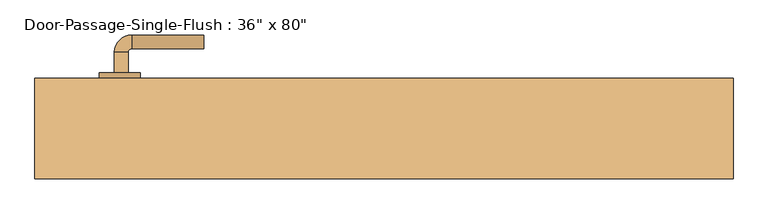
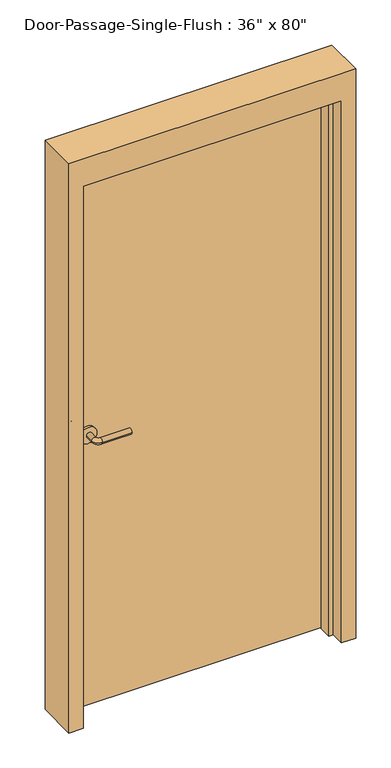
"""IFC4 building model written with IfcOpenShell, lengths in millimetres: door geometry."""

from ifc_helpers import new_model, si_unit, point, frame, frame_2d, origin, origin_with_axes, place, context, project, spatial, polyline, circle_curve, ellipse_curve, trimmed, segment, composite_curve, outline, extrude, faceted_brep, source, transform, mapped, element, save
from ifc_brep_helpers import plane_surface, cylinder_surface, revolved_surface, advanced_brep


def door_64a1d9e0(model_context):
    return source(origin(), model_context, "Body", "SolidModel", [
        advanced_brep(
        [(-392.190625, 17.4, 1016.0), (-372.190625, 17.4, 1016.0), (-372.190625, -12.6, 1016.0), (-392.190625, -12.6, 1016.0), (-367.190625, -17.6, 1016.0), (-367.190625, -37.6, 1016.0), (-262.190625, -37.6, 1016.0), (-262.190625, -17.6, 1016.0)],
        [
            (0, 1, circle_curve(frame((-382.190625, 17.4, 1016.0), z_axis=(0.0, 1.0, 0.0), x_axis=(1.0, 0.0, 0.0)), 10.0)),
            (1, 0, circle_curve(frame((-382.190625, 17.4, 1016.0), z_axis=(0.0, 1.0, 0.0), x_axis=(1.0, 0.0, 0.0)), 10.0)),
            (1, 2),
            (2, 3, circle_curve(frame((-382.190625, -12.6, 1016.0), z_axis=(0.0, 1.0, 0.0), x_axis=(1.0, 0.0, 0.0)), 10.0)),
            (3, 0),
            (3, 2, circle_curve(frame((-382.190625, -12.6, 1016.0), z_axis=(0.0, 1.0, 0.0), x_axis=(1.0, 0.0, 0.0)), 10.0)),
            (4, 5, circle_curve(frame((-367.190625, -27.6, 1016.0), z_axis=(-1.0, 0.0, 0.0), x_axis=(0.0, 1.0, 0.0)), 10.0)),
            (5, 3, circle_curve(frame((-367.190625, -12.6, 1016.0), z_axis=(0.0, 0.0, -1.0), x_axis=(-1.0, 0.0, 0.0)), 25.0)),
            (2, 4, circle_curve(frame((-367.190625, -12.6, 1016.0), z_axis=(0.0, 0.0, 1.0), x_axis=(-1.0, 0.0, 0.0)), 5.0)),
            (5, 4, circle_curve(frame((-367.190625, -27.6, 1016.0), z_axis=(-1.0, 0.0, 0.0), x_axis=(0.0, 1.0, 0.0)), 10.0)),
            (6, 7, circle_curve(frame((-262.190625, -27.6, 1016.0), z_axis=(1.0, 0.0, 0.0), x_axis=(0.0, 1.0, 0.0)), 10.0)),
            (7, 6, circle_curve(frame((-262.190625, -27.6, 1016.0), z_axis=(1.0, 0.0, 0.0), x_axis=(0.0, 1.0, 0.0)), 10.0)),
            (4, 7),
            (6, 5),
        ],
        [
            plane_surface(frame((-382.190625, 17.4, 1016.0), z_axis=(0.0, 1.0, 0.0), x_axis=(0.0, 0.0, 1.0))),
            cylinder_surface(frame((-382.190625, 17.4, 1016.0), z_axis=(0.0, 1.0, 0.0), x_axis=(1.0, 0.0, 0.0)), 10.0),
            revolved_surface(trimmed(ellipse_curve(frame((-382.190625, -12.6, 1016.0), z_axis=(0.0, -1.0, 0.0), x_axis=(1.0, 0.0, 0.0)), 10.0, 10.0), [point((-392.190625, -12.6, 1016.0))], [point((-372.190625, -12.6, 1016.0))], True, "CARTESIAN"), (-367.190625, -12.6, 1016.0), (0.0, 0.0, -1.0)),
            revolved_surface(trimmed(ellipse_curve(frame((-382.190625, -12.6, 1016.0), z_axis=(0.0, -1.0, 0.0), x_axis=(1.0, 0.0, 0.0)), 10.0, 10.0), [point((-372.190625, -12.6, 1016.0))], [point((-392.190625, -12.6, 1016.0))], True, "CARTESIAN"), (-367.190625, -12.6, 1016.0), (0.0, 0.0, -1.0)),
            plane_surface(frame((-262.190625, -27.6, 1016.0), z_axis=(1.0, 0.0, 0.0), x_axis=(0.0, 0.0, 1.0))),
            cylinder_surface(frame((-367.190625, -27.6, 1016.0), z_axis=(-1.0, 0.0, 0.0), x_axis=(0.0, 1.0, 0.0)), 10.0),
        ],
        [
            (0, [[1, 2]]),
            (1, [[3, 4, 5, -2]]),
            (1, [[-5, 6, -3, -1]]),
            (2, [[7, 8, -4, 9]]),
            (3, [[10, -9, -6, -8]]),
            (4, [[11, 12]]),
            (5, [[13, -11, 14, -7]]),
            (5, [[-14, -12, -13, -10]]),
        ],
    ),
        extrude(outline(composite_curve([segment(trimmed(circle_curve(frame_2d((1016.0, -384.690625)), 30.0), [point((1016.0, -414.690625))], [point((1016.0, -354.690625))], False, "CARTESIAN"), True, "CONTINUOUS"), segment(trimmed(circle_curve(frame_2d((1016.0, -384.690625)), 30.0), [point((1016.0, -354.690625))], [point((1016.0, -414.690625))], False, "CARTESIAN"), True, "CONTINUOUS")], self_intersect=False)), frame((0.0, 17.4, 0.0), z_axis=(0.0, 1.0, 0.0), x_axis=(0.0, 0.0, 1.0)), (0.0, 0.0, 1.0), 8.0),
        advanced_brep(
        [(-392.190625, 77.85, 1016.0), (-372.190625, 77.85, 1016.0), (-392.190625, 107.85, 1016.0), (-372.190625, 107.85, 1016.0), (-367.190625, 112.85, 1016.0), (-367.190625, 132.85, 1016.0), (-262.190625, 132.85, 1016.0), (-262.190625, 112.85, 1016.0)],
        [
            (0, 1, circle_curve(frame((-382.190625, 77.85, 1016.0), z_axis=(0.0, -1.0, 0.0), x_axis=(1.0, 0.0, 0.0)), 10.0)),
            (1, 0, circle_curve(frame((-382.190625, 77.85, 1016.0), z_axis=(0.0, -1.0, 0.0), x_axis=(1.0, 0.0, 0.0)), 10.0)),
            (0, 2),
            (2, 3, circle_curve(frame((-382.190625, 107.85, 1016.0), z_axis=(0.0, -1.0, 0.0), x_axis=(1.0, 0.0, 0.0)), 10.0)),
            (3, 1),
            (3, 2, circle_curve(frame((-382.190625, 107.85, 1016.0), z_axis=(0.0, -1.0, 0.0), x_axis=(1.0, 0.0, 0.0)), 10.0)),
            (4, 3, circle_curve(frame((-367.190625, 107.85, 1016.0), z_axis=(0.0, 0.0, 1.0), x_axis=(-1.0, 0.0, 0.0)), 5.0)),
            (2, 5, circle_curve(frame((-367.190625, 107.85, 1016.0), z_axis=(0.0, 0.0, -1.0), x_axis=(-1.0, 0.0, 0.0)), 25.0)),
            (5, 4, circle_curve(frame((-367.190625, 122.85, 1016.0), z_axis=(-1.0, 0.0, 0.0), x_axis=(0.0, -1.0, 0.0)), 10.0)),
            (4, 5, circle_curve(frame((-367.190625, 122.85, 1016.0), z_axis=(-1.0, 0.0, 0.0), x_axis=(0.0, -1.0, 0.0)), 10.0)),
            (6, 7, circle_curve(frame((-262.190625, 122.85, 1016.0), z_axis=(1.0, 0.0, 0.0), x_axis=(0.0, -1.0, 0.0)), 10.0)),
            (7, 6, circle_curve(frame((-262.190625, 122.85, 1016.0), z_axis=(1.0, 0.0, 0.0), x_axis=(0.0, -1.0, 0.0)), 10.0)),
            (5, 6),
            (7, 4),
        ],
        [
            plane_surface(frame((-382.190625, 77.85, 1016.0), z_axis=(0.0, -1.0, 0.0), x_axis=(0.0, 0.0, 1.0))),
            cylinder_surface(frame((-382.190625, 77.85, 1016.0), z_axis=(0.0, -1.0, 0.0), x_axis=(1.0, 0.0, 0.0)), 10.0),
            revolved_surface(trimmed(ellipse_curve(frame((-382.190625, 107.85, 1016.0), z_axis=(0.0, -1.0, 0.0), x_axis=(1.0, 0.0, 0.0)), 10.0, 10.0), [point((-392.190625, 107.85, 1016.0))], [point((-372.190625, 107.85, 1016.0))], True, "CARTESIAN"), (-367.190625, 107.85, 1016.0), (0.0, 0.0, -1.0)),
            revolved_surface(trimmed(ellipse_curve(frame((-382.190625, 107.85, 1016.0), z_axis=(0.0, -1.0, 0.0), x_axis=(1.0, 0.0, 0.0)), 10.0, 10.0), [point((-372.190625, 107.85, 1016.0))], [point((-392.190625, 107.85, 1016.0))], True, "CARTESIAN"), (-367.190625, 107.85, 1016.0), (0.0, 0.0, -1.0)),
            plane_surface(frame((-262.190625, 122.85, 1016.0), z_axis=(1.0, 0.0, 0.0), x_axis=(0.0, 0.0, 1.0))),
            cylinder_surface(frame((-367.190625, 122.85, 1016.0), z_axis=(-1.0, 0.0, 0.0), x_axis=(0.0, -1.0, 0.0)), 10.0),
        ],
        [
            (0, [[1, 2]]),
            (1, [[-1, 3, 4, 5]]),
            (1, [[-2, -5, 6, -3]]),
            (2, [[7, -4, 8, 9]]),
            (3, [[-8, -6, -7, 10]]),
            (4, [[11, 12]]),
            (5, [[-9, 13, -12, 14]]),
            (5, [[-10, -14, -11, -13]]),
        ],
    ),
        extrude(outline(composite_curve([segment(trimmed(circle_curve(frame_2d((1016.0, -384.690625)), 30.0), [point((1016.0, -414.690625))], [point((1016.0, -354.690625))], False, "CARTESIAN"), True, "CONTINUOUS"), segment(trimmed(circle_curve(frame_2d((1016.0, -384.690625)), 30.0), [point((1016.0, -354.690625))], [point((1016.0, -414.690625))], False, "CARTESIAN"), True, "CONTINUOUS")], self_intersect=False)), frame((0.0, 69.85, 0.0), z_axis=(0.0, 1.0, 0.0), x_axis=(0.0, 0.0, 1.0)), (0.0, 0.0, 1.0), 8.0),
        faceted_brep([(457.2, 20.6375, 0.0), (457.2, 69.85, 0.0), (508.0, 69.85, 0.0), (508.0, -76.2, 0.0), (457.2, -76.2, 0.0), (457.2, -26.9875, 0.0), (441.325, -26.9875, 0.0), (441.325, 20.6375, 0.0), (457.2, 20.6375, 2032.0), (457.2, 69.85, 2032.0), (-457.2, 69.85, 2032.0), (-457.2, 69.85, 0.0), (-508.0, 69.85, 0.0), (-508.0, 69.85, 2133.6), (508.0, 69.85, 2133.6), (508.0, -76.2, 2133.6), (-508.0, -76.2, 2133.6), (-508.0, -76.2, 0.0), (-457.2, -76.2, 0.0), (-457.2, -76.2, 2032.0), (457.2, -76.2, 2032.0), (457.2, -26.9875, 2032.0), (-457.2, -26.9875, 2032.0), (-457.2, -26.9875, 0.0), (-441.325, -26.9875, 0.0), (-441.325, -26.9875, 2016.125), (441.325, -26.9875, 2016.125), (441.325, 20.6375, 2016.125), (-441.325, 20.6375, 2016.125), (-441.325, 20.6375, 0.0), (-457.2, 20.6375, 0.0), (-457.2, 20.6375, 2032.0)], [[[0, 1, 2, 3, 4, 5, 6, 7]], [[1, 0, 8, 9]], [[2, 1, 9, 10, 11, 12, 13, 14]], [[3, 2, 14, 15]], [[4, 3, 15, 16, 17, 18, 19, 20]], [[5, 4, 20, 21]], [[6, 5, 21, 22, 23, 24, 25, 26]], [[7, 6, 26, 27]], [[0, 7, 27, 28, 29, 30, 31, 8]], [[9, 8, 31, 10]], [[20, 19, 22, 21]], [[26, 25, 28, 27]], [[12, 11, 30, 29, 24, 23, 18, 17]], [[11, 10, 31, 30]], [[13, 12, 17, 16]], [[19, 18, 23, 22]], [[25, 24, 29, 28]], [[15, 14, 13, 16]]]),
        extrude(outline(polyline([(457.2, 25.4), (-457.2, 25.4), (-457.2, 69.85), (457.2, 69.85), (457.2, 25.4)])), origin_with_axes(), (0.0, 0.0, 1.0), 2032.0),
    ])


if __name__ == "__main__":
    model = new_model("IFC4")
    model_context = context("Model", 3, world=origin())
    ifc_project = project(units=[si_unit("LENGTHUNIT", "METRE", prefix="MILLI")], contexts=[model_context])
    site = spatial("IfcSite", under=ifc_project)
    building = spatial("IfcBuilding", under=site)
    placement = place(None, origin())
    door_shape = door_64a1d9e0(model_context)
    element("IfcDoor", 1, ObjectType="Door-Passage-Single-Flush : 36\" x 80\"", at=placement, inside=building, context=model_context, shape_type="MappedRepresentation", body=[
        mapped(door_shape, transform((0.0, 0.0, 0.0), x_axis=(1.0, 0.0, 0.0), y_axis=(0.0, 1.0, 0.0), z_axis=(0.0, 0.0, 1.0))),
    ])
    save(model, "model.ifc")

# Revit data of these elements
# Type "Door-Passage-Single-Flush : 36\" x 80\""
#   Type Mark = "16"
#   Assembly Code = "B2030200"
#   Analytic Construction = "Wooden"
#   Thickness = 0' - 1 3/4"
#   Thermal Resistance (R) = 0.455703 (m²·K)/W
#   Swing Angle [instance default] = 90.00°
#   Strike Height = 3' - 4"
#   Rough Width [instance default] = 3' - 4"
#   Rough Height [instance default] = 7' - 0"
#   MF Opening Height [instance default] = 0' - 4"
#   MF Opening Width [instance default] = 0' - 4"
#   Inset Calculate [instance default] = 0' - 4"
#   Masonry Inset [instance default] = 0' - 1"
#   Height = 6' - 8"
#   Width = 3' - 0"
#   Heat Transfer Coefficient (U) = 2.19465 W/(m²·K)
#   Masonry Frame Depth = 0' - 5 3/4"
#   Masonry Frame [instance default] = yes
#   Function = 1
#   Dry Wall Frame [instance default] = no
#   Panel Material = Wood - Birch
#   Frame Material = Metal - Paint Finish - Grey
#   Door Handle Material = Aluminum
#   Visual Light Transmittance = 0
#   Solar Heat Gain Coefficient = 0
#   Wall Closure = (empty or 0)
# Element 1 (IfcDoor, "Door-Passage-Single-Flush : 36\" x 80\"")
#   Inset Calculate = 0' - 2 1/2"
#   Masonry Inset = -0' - 0 1/2"
#   Materials on its faces: "Aluminum", "Metal - Paint Finish - Grey", "Wood - Birch"
# Materials
#   "Wood - Birch": class "Wood", colour RGB 166 116 52, transparency 0, Cost = 0
#   "Metal - Paint Finish - Grey": class "Paint", colour RGB 104 104 104, transparency 0, Cost = 0
#   "Aluminum": class "Metal", colour RGB 247 247 247, transparency 0, Description = "Aluminum 6061", Cost = 0
